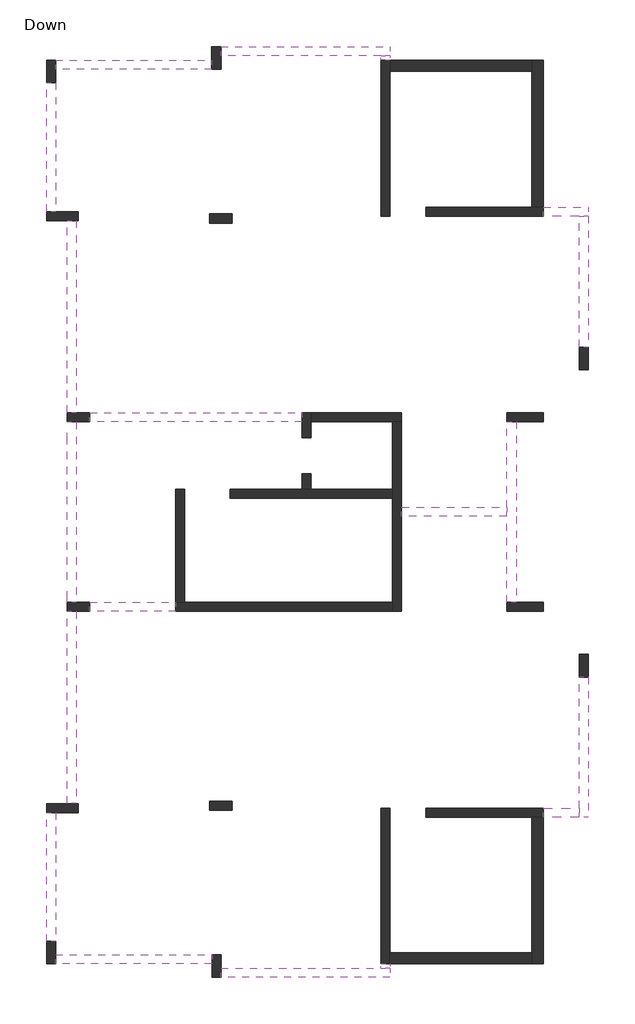
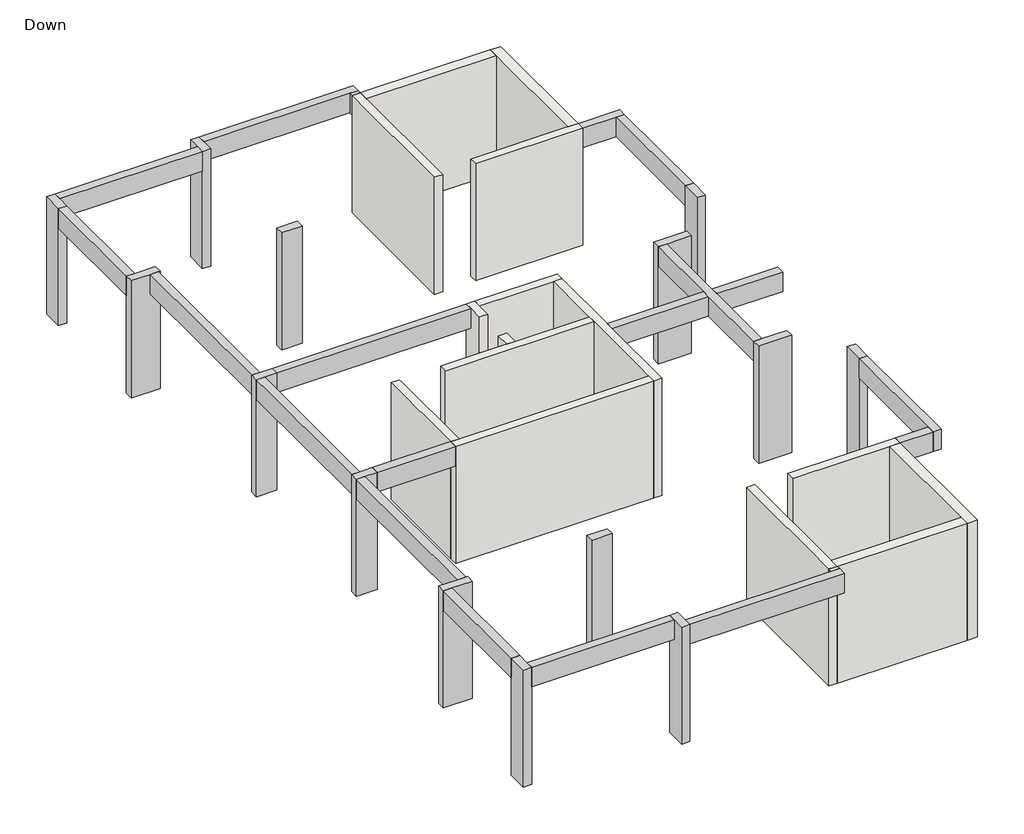
# One storey: 19 beams, 15 walls, 14 columns.
# Revit data of these elements (continued)
# Element 44 (IfcWall, "20") (continued)
#   SOFiSTiK_EdgeZones = "W11"
#   SOFiSTiK_AMG_Comments = ""
#   Top Offset = 0 cm
#   Base Offset = 0 cm
#   wall height = 300 cm
#   SOFiSTiK_AMG_Scheduled = yes
#   SOFiSTiK_AMG_Adjusted = yes
#   Phase Created = New Construction
#   Base Constraint = Down
#   Top Constraint = Typical Floor
#   Materials on its faces: "Concrete"
# Element 45 (IfcWall, "25")
#   Comments = ""
#   Mark = "W12"
#   SOFiSTiK_EdgeZones = "W12"
#   SOFiSTiK_AMG_Comments = ""
#   Top Offset = 0 cm
#   Base Offset = 0 cm
#   wall height = 300 cm
#   SOFiSTiK_AMG_Scheduled = yes
#   SOFiSTiK_AMG_Adjusted = yes
#   Phase Created = New Construction
#   Base Constraint = Down
#   Top Constraint = Typical Floor
#   Materials on its faces: "Concrete"
# Element 46 (IfcWall, "25")
#   Comments = ""
#   Mark = "W13"
#   SOFiSTiK_EdgeZones = "W13"
#   SOFiSTiK_AMG_Comments = ""
#   Top Offset = 0 cm
#   Base Offset = 0 cm
#   wall height = 300 cm
#   SOFiSTiK_AMG_Scheduled = yes
#   SOFiSTiK_AMG_Adjusted = yes
#   Phase Created = New Construction
#   Base Constraint = Down
#   Top Constraint = Typical Floor
#   Materials on its faces: "Concrete"
# Element 47 (IfcWall, "25")
#   Comments = ""
#   Mark = "W14"
#   SOFiSTiK_EdgeZones = "W14"
#   SOFiSTiK_AMG_Comments = ""
#   Top Offset = 0 cm
#   Base Offset = 0 cm
#   wall height = 300 cm
#   SOFiSTiK_AMG_Scheduled = yes
#   SOFiSTiK_AMG_Adjusted = yes
#   Phase Created = New Construction
#   Base Constraint = Down
#   Top Constraint = Typical Floor
#   Materials on its faces: "Concrete"
# Element 48 (IfcWall, "25")
#   Comments = ""
#   Mark = "W15"
#   SOFiSTiK_EdgeZones = "W15"
#   SOFiSTiK_AMG_Comments = ""
#   Top Offset = 0 cm
#   Base Offset = 0 cm
#   wall height = 300 cm
#   SOFiSTiK_AMG_Scheduled = yes
#   SOFiSTiK_AMG_Adjusted = yes
#   Phase Created = New Construction
#   Base Constraint = Down
#   Top Constraint = Typical Floor
#   Materials on its faces: "Concrete"
# Materials
#   "Concrete": class "Concrete", colour RGB 192 192 192, transparency 0, Keynote = "01000", Description = "Cast-in-place concrete", Cost = 0
